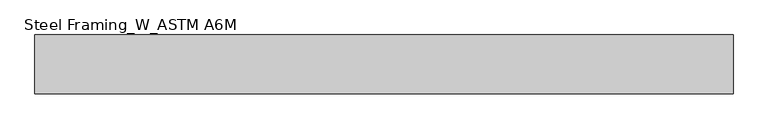
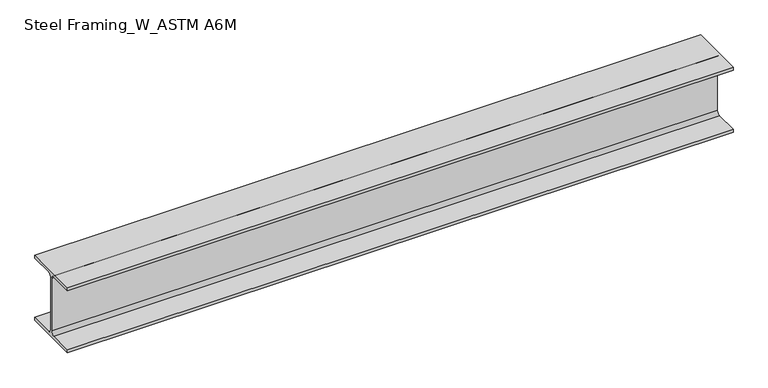
"""IFC4 building model written with IfcOpenShell, lengths in millimetres: beam geometry, Steel Framing_W_ASTM A6M : H_SB_AR_S02_W250x49.1_RCG1."""

import ifcopenshell
import ifcopenshell.guid

model = None  # the IFC model being written
_history = None  # IfcOwnerHistory: only IFC2X3 demands one
_inside = {}  # id of a spatial element -> (the spatial element, [elements in it])
_under = {}  # id of a project, library or spatial element -> (it, [spatial elements below it])
_declared = {}  # id of a project -> (the project, [libraries it declares])
_typed = {}  # id of a type object -> (the type object, [elements of that type])
_made_of = {}  # id of a material, layer set ... -> (it, [elements and type objects made of it])


def new_model(schema):
    """Start an empty IFC model of exactly this schema.

    Asked for "IFC4X3", IfcOpenShell would pick the latest addendum, in which some entities
    have other attributes; the version numbers below select the first issue.
    IFC2X3 requires an IfcOwnerHistory on every rooted entity: one is made here for all.
    """
    global model, _history
    if schema == "IFC4X3":
        model = ifcopenshell.file(schema_version=(4, 3, 0, 0))
    else:
        model = ifcopenshell.file(schema=schema)
    _inside.clear()
    _under.clear()
    _declared.clear()
    _typed.clear()
    _made_of.clear()
    _history = None
    if model.schema == "IFC2X3":
        org = make("IfcOrganization", Name="unknown")
        user = make(
            "IfcPersonAndOrganization",
            ThePerson=make("IfcPerson", FamilyName="unknown"),
            TheOrganization=org,
        )
        app = make(
            "IfcApplication",
            ApplicationDeveloper=org,
            Version="unknown",
            ApplicationFullName="unknown",
            ApplicationIdentifier="unknown",
        )
        _history = make(
            "IfcOwnerHistory",
            OwningUser=user,
            OwningApplication=app,
            ChangeAction="ADDED",
            CreationDate=0,
        )
    return model


def make(cls, **values):
    """One entity of the class cls with the attributes given. An attribute that is None is left unset."""
    return model.create_entity(
        cls, **{name: value for name, value in values.items() if value is not None}
    )


def rooted(cls, **values):
    """An entity with a GlobalId (a new one), such as an element, a storey or a relation."""
    return make(cls, GlobalId=ifcopenshell.guid.new(), OwnerHistory=_history, **values)


def si_unit(unit_type, name, prefix=None):
    """IfcSIUnit, for example si_unit("LENGTHUNIT", "METRE", prefix="MILLI")."""
    return make("IfcSIUnit", UnitType=unit_type, Prefix=prefix, Name=name)


def assignment(units):
    """IfcUnitAssignment: the units of a project."""
    return None if units is None else make("IfcUnitAssignment", Units=units)


def point(xyz):
    """IfcCartesianPoint."""
    return None if xyz is None else make("IfcCartesianPoint", Coordinates=xyz)


def direction(xyz):
    """IfcDirection."""
    return None if xyz is None else make("IfcDirection", DirectionRatios=xyz)


def frame(location, z_axis=None, x_axis=None):
    """IfcAxis2Placement3D, a coordinate frame: its origin and axes. An axis left out is left unset."""
    return make(
        "IfcAxis2Placement3D",
        Location=point(location),
        Axis=direction(z_axis),
        RefDirection=direction(x_axis),
    )


def frame_2d(location, x_axis=None):
    """IfcAxis2Placement2D, a coordinate frame in the plane: its origin and x axis."""
    return make(
        "IfcAxis2Placement2D", Location=point(location), RefDirection=direction(x_axis)
    )


def origin():
    """The frame at (0, 0, 0) with its axes left unset."""
    return frame((0.0, 0.0, 0.0))


def place(relative_to, where):
    """IfcLocalPlacement: puts the frame where relative to a parent placement (None: the world)."""
    return make(
        "IfcLocalPlacement", PlacementRelTo=relative_to, RelativePlacement=where
    )


def context(
    kind, dimensions, precision=None, world=None, true_north=None, identifier=None
):
    """IfcGeometricRepresentationContext, for example the 3D "Model" context."""
    return make(
        "IfcGeometricRepresentationContext",
        ContextIdentifier=identifier,
        ContextType=kind,
        CoordinateSpaceDimension=dimensions,
        Precision=precision,
        WorldCoordinateSystem=world,
        TrueNorth=true_north,
    )


def project(units=None, contexts=None):
    """IfcProject with its units and contexts."""
    return rooted(
        "IfcProject",
        Name="project",
        RepresentationContexts=contexts,
        UnitsInContext=assignment(units),
    )


def spatial(cls, under=None, at=None, **own):
    """A site, building, storey or space (cls), placed at a placement, below another one or the project."""
    s = rooted(cls, ObjectPlacement=at, **own)
    if under is not None:
        _under.setdefault(under.id(), (under, []))[1].append(s)
    return s


def polyline(points):
    """IfcPolyline through the points."""
    return make("IfcPolyline", Points=[point(p) for p in points])


def circle_curve(where, radius):
    """IfcCircle in the frame where."""
    return make("IfcCircle", Position=where, Radius=radius)


def trimmed(basis, trim1, trim2, sense, master):
    """IfcTrimmedCurve: the piece of a basis curve between two trims."""
    return make(
        "IfcTrimmedCurve",
        BasisCurve=basis,
        Trim1=trim1,
        Trim2=trim2,
        SenseAgreement=sense,
        MasterRepresentation=master,
    )


def segment(curve, same_sense, transition):
    """IfcCompositeCurveSegment."""
    return make(
        "IfcCompositeCurveSegment",
        Transition=transition,
        SameSense=same_sense,
        ParentCurve=curve,
    )


def composite_curve(segments, self_intersect=None):
    """IfcCompositeCurve: segments joined end to end."""
    return make("IfcCompositeCurve", Segments=segments, SelfIntersect=self_intersect)


def outline(outer, holes=None, kind="AREA"):
    """IfcArbitraryClosedProfileDef: a profile drawn as a closed curve; with holes, ...WithVoids."""
    if holes is None:
        return make("IfcArbitraryClosedProfileDef", ProfileType=kind, OuterCurve=outer)
    return make(
        "IfcArbitraryProfileDefWithVoids",
        ProfileType=kind,
        OuterCurve=outer,
        InnerCurves=holes,
    )


def extrude(swept, where, along, depth):
    """IfcExtrudedAreaSolid: the profile swept, set in the frame where, extruded along a direction by depth."""
    return make(
        "IfcExtrudedAreaSolid",
        SweptArea=swept,
        Position=where,
        ExtrudedDirection=direction(along),
        Depth=depth,
    )


def shape(context_of_items, identifier, shape_type, items):
    """IfcShapeRepresentation: the items that make up one representation, for example the "Body"."""
    return make(
        "IfcShapeRepresentation",
        ContextOfItems=context_of_items,
        RepresentationIdentifier=identifier,
        RepresentationType=shape_type,
        Items=items,
    )


def source(mapping_origin, context_of_items, identifier, shape_type, items):
    """IfcRepresentationMap: a shape defined once, which mapped items show again and again."""
    return make(
        "IfcRepresentationMap",
        MappingOrigin=mapping_origin,
        MappedRepresentation=shape(context_of_items, identifier, shape_type, items),
    )


def transform(
    local_origin,
    x_axis=None,
    y_axis=None,
    z_axis=None,
    scale=None,
    scale2=None,
    scale3=None,
    uniform=True,
):
    """IfcCartesianTransformationOperator3D, or its non-uniform kind. x_axis, y_axis, z_axis: its Axis1, 2, 3."""
    if uniform:
        return make(
            "IfcCartesianTransformationOperator3D",
            Axis1=direction(x_axis),
            Axis2=direction(y_axis),
            LocalOrigin=point(local_origin),
            Scale=scale,
            Axis3=direction(z_axis),
        )
    return make(
        "IfcCartesianTransformationOperator3DnonUniform",
        Axis1=direction(x_axis),
        Axis2=direction(y_axis),
        LocalOrigin=point(local_origin),
        Scale=scale,
        Axis3=direction(z_axis),
        Scale2=scale2,
        Scale3=scale3,
    )


def mapped(mapping_source, mapping_target):
    """IfcMappedItem: shows the shape of a source again, moved by a transform."""
    return make(
        "IfcMappedItem", MappingSource=mapping_source, MappingTarget=mapping_target
    )


def made_of(thing, what):
    """Note that an element or type object is made of a material, layer set ...; save() writes the relation."""
    if what is not None:
        _made_of.setdefault(what.id(), (what, []))[1].append(thing)
    return thing


def element(
    cls,
    number,
    at=None,
    inside=None,
    cuts=None,
    type_object=None,
    material=None,
    context=None,
    identifier="Body",
    shape_type=None,
    held_by="IfcProductDefinitionShape",
    body=None,
    shapes=None,
    **own,
):
    """One element of the class cls, such as IfcWall. Its Tag is "e" and its number.

    at: its placement. inside: the storey or other place that contains it. cuts: it is an
    opening in that element (IfcRelVoidsElement). A single representation is given by context,
    identifier, shape_type and body (its items); several are given by shapes. held_by: the class
    of the entity that holds the representations. save() writes the other relations.
    """
    e = rooted(cls, Tag="e%d" % number, ObjectPlacement=at, **own)
    if body is not None:
        shapes = [shape(context, identifier, shape_type, body)]
    if shapes is not None:
        e.Representation = make(held_by, Representations=shapes)
    if inside is not None:
        _inside.setdefault(inside.id(), (inside, []))[1].append(e)
    if cuts is not None:
        rooted(
            "IfcRelVoidsElement", RelatingBuildingElement=cuts, RelatedOpeningElement=e
        )
    if type_object is not None:
        _typed.setdefault(type_object.id(), (type_object, []))[1].append(e)
    return made_of(e, material)


def aggregate(whole, parts):
    """IfcRelAggregates: a whole, such as a stair, and the parts it consists of."""
    return rooted("IfcRelAggregates", RelatingObject=whole, RelatedObjects=parts)


def save(model, path):
    """Write the relations noted so far, then the file.

    IfcRelAggregates (storeys below a building ...), IfcRelContainedInSpatialStructure (elements
    in a storey), IfcRelDefinesByType, IfcRelAssociatesMaterial and IfcRelDeclares: one each for
    every whole, place, type object, material and project.
    """
    for whole, parts in _under.values():
        aggregate(whole, parts)
    for where, things in _inside.values():
        rooted(
            "IfcRelContainedInSpatialStructure",
            RelatedElements=things,
            RelatingStructure=where,
        )
    for kind, things in _typed.values():
        rooted("IfcRelDefinesByType", RelatedObjects=things, RelatingType=kind)
    for what, things in _made_of.values():
        rooted("IfcRelAssociatesMaterial", RelatedObjects=things, RelatingMaterial=what)
    for by, libraries in _declared.values():
        rooted("IfcRelDeclares", RelatingContext=by, RelatedDefinitions=libraries)
    model.write(path)


def steel_framing_w_astm_a6m_c3bcebff(model_context):
    return source(origin(), model_context, "Body", "SweptSolid", [
        extrude(outline(composite_curve([segment(polyline([(101.0, -112.5), (101.0, -123.5), (-101.0, -123.5), (-101.0, -112.5), (-16.385, -112.5)]), True, "CONTINUOUS"), segment(trimmed(circle_curve(frame_2d((-16.385, -99.8)), 12.7), [point((-16.385, -112.5))], [point((-3.685, -99.8))], True, "CARTESIAN"), True, "CONTINUOUS"), segment(polyline([(-3.685, -99.8), (-3.685, 99.8)]), True, "CONTINUOUS"), segment(trimmed(circle_curve(frame_2d((-16.385, 99.8)), 12.7), [point((-3.685, 99.8))], [point((-16.385, 112.5))], True, "CARTESIAN"), True, "CONTINUOUS"), segment(polyline([(-16.385, 112.5), (-101.0, 112.5), (-101.0, 123.5), (101.0, 123.5), (101.0, 112.5), (16.385, 112.5)]), True, "CONTINUOUS"), segment(trimmed(circle_curve(frame_2d((16.385, 99.8)), 12.7), [point((16.385, 112.5))], [point((3.685, 99.8))], True, "CARTESIAN"), True, "CONTINUOUS"), segment(polyline([(3.685, 99.8), (3.685, -99.8)]), True, "CONTINUOUS"), segment(trimmed(circle_curve(frame_2d((16.385, -99.8)), 12.7), [point((3.685, -99.8))], [point((16.385, -112.5))], True, "CARTESIAN"), True, "CONTINUOUS"), segment(polyline([(16.385, -112.5), (101.0, -112.5)]), True, "CONTINUOUS")], self_intersect=False)), frame((-1243.5, 0.0, 0.0), z_axis=(1.0, 0.0, 0.0), x_axis=(0.0, 1.0, 0.0)), (0.0, 0.0, 1.0), 2391.9525253),
    ])


if __name__ == "__main__":
    model = new_model("IFC4")
    model_context = context("Model", 3, world=origin())
    ifc_project = project(units=[si_unit("LENGTHUNIT", "METRE", prefix="MILLI")], contexts=[model_context])
    site = spatial("IfcSite", under=ifc_project)
    building = spatial("IfcBuilding", under=site)
    placement = place(None, origin())
    steel_framing_w_astm_a6m_shape = steel_framing_w_astm_a6m_c3bcebff(model_context)
    element("IfcBeam", 1, ObjectType="Steel Framing_W_ASTM A6M : H_SB_AR_S02_W250x49.1_RCG1", at=placement, inside=building, context=model_context, shape_type="MappedRepresentation", body=[
        mapped(steel_framing_w_astm_a6m_shape, transform((0.0, 0.0, 0.0), x_axis=(1.0, 0.0, 0.0), y_axis=(0.0, 1.0, 0.0), z_axis=(0.0, 0.0, 1.0))),
    ])
    save(model, "model.ifc")

# Revit data of these elements
# Type "Steel Framing_W_ASTM A6M : H_SB_AR_S02_W250x49.1_RCG1"
#   Type Mark = "RCG1"
#   Section Name Key = "W10x33"
#   Width = 20.2 cm
#   Web Thickness = 0.737 cm
#   Web Fillet = 1.27 cm
#   Warping Constant = 212000.0 cm⁶
#   Torsional Moment of Inertia = 24.30 cm⁴
#   Section Area = 62.6 cm²
#   Plastic Modulus weak axis = 229.0 cm³
#   Plastic Modulus strong axis = 636.0 cm³
#   Perimeter = 1.27 m²/m
#   Nominal Weight = 49.10 kgf/m
#   Moment of Inertia weak axis = 1520.00 cm⁴
#   Moment of Inertia strong axis = 7120.00 cm⁴
#   Height = 24.7 cm
#   Flange Thickness = 1.1 cm
#   Elastic Modulus weak axis = 151.0 cm³
#   Elastic Modulus strong axis = 574.0 cm³
#   Centroid Vertical = 12.35 cm
#   Centroid Horizontal = 10.1 cm
#   Length [instance default] = 1500 mm
#   Structural Material [instance default] = Steel, 45-345
#   Bolt Spacing = 0
#   Assembly Code = ""
# Element 1 (IfcBeam, "Steel Framing_W_ASTM A6M : H_SB_AR_S02_W250x49.1_RCG1")
#   Materials on its faces: "Steel, 45-345"
# Materials
#   "Steel, 45-345": class "Metal", colour RGB 189 187 185, transparency 0, Description = "Steel 345 MPa", Cost = 0
